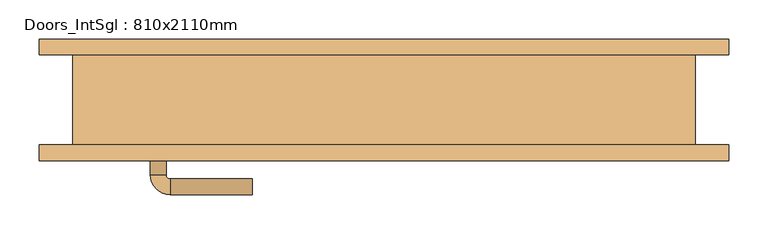
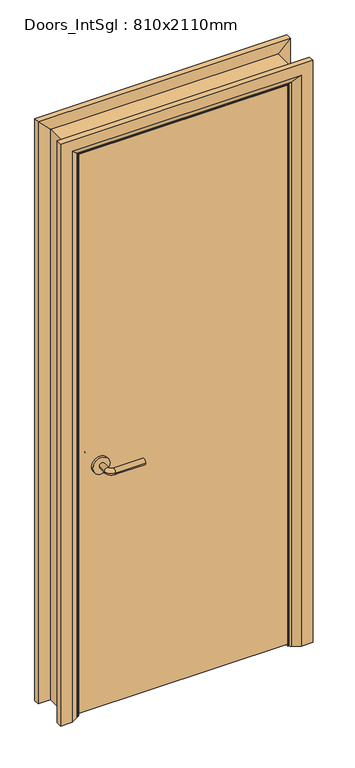
"""IFC4 building model written with IfcOpenShell, lengths in millimetres: door geometry, Doors_IntSgl : 810x2110mm."""

from ifc_helpers import new_model, si_unit, point, frame, frame_2d, origin, place, context, project, spatial, polyline, circle_curve, ellipse_curve, trimmed, segment, composite_curve, outline, extrude, faceted_brep, source, transform, mapped, element, save
from ifc_brep_helpers import plane_surface, cylinder_surface, revolved_surface, advanced_brep


def doors_intsgl_810x2110mm_b7c9fbf7(model_context):
    return source(origin(), model_context, "Body", "SolidModel", [
        advanced_brep(
        [(-298.0, -11.5, 900.0), (-278.0, -11.5, 900.0), (-298.0, 18.5, 900.0), (-278.0, 18.5, 900.0), (-273.0, 23.5, 900.0), (-273.0, 43.5, 900.0), (-168.0, 43.5, 900.0), (-168.0, 23.5, 900.0)],
        [
            (0, 1, circle_curve(frame((-288.0, -11.5, 900.0), z_axis=(0.0, -1.0, 0.0), x_axis=(1.0, 0.0, 0.0)), 10.0)),
            (1, 0, circle_curve(frame((-288.0, -11.5, 900.0), z_axis=(0.0, -1.0, 0.0), x_axis=(1.0, 0.0, 0.0)), 10.0)),
            (0, 2),
            (2, 3, circle_curve(frame((-288.0, 18.5, 900.0), z_axis=(0.0, -1.0, 0.0), x_axis=(1.0, 0.0, 0.0)), 10.0)),
            (3, 1),
            (3, 2, circle_curve(frame((-288.0, 18.5, 900.0), z_axis=(0.0, -1.0, 0.0), x_axis=(1.0, 0.0, 0.0)), 10.0)),
            (4, 3, circle_curve(frame((-273.0, 18.5, 900.0), z_axis=(0.0, 0.0, 1.0), x_axis=(-1.0, 0.0, 0.0)), 5.0)),
            (2, 5, circle_curve(frame((-273.0, 18.5, 900.0), z_axis=(0.0, 0.0, -1.0), x_axis=(-1.0, 0.0, 0.0)), 25.0)),
            (5, 4, circle_curve(frame((-273.0, 33.5, 900.0), z_axis=(-1.0, 0.0, 0.0), x_axis=(0.0, -1.0, 0.0)), 10.0)),
            (4, 5, circle_curve(frame((-273.0, 33.5, 900.0), z_axis=(-1.0, 0.0, 0.0), x_axis=(0.0, -1.0, 0.0)), 10.0)),
            (6, 7, circle_curve(frame((-168.0, 33.5, 900.0), z_axis=(1.0, 0.0, 0.0), x_axis=(0.0, -1.0, 0.0)), 10.0)),
            (7, 6, circle_curve(frame((-168.0, 33.5, 900.0), z_axis=(1.0, 0.0, 0.0), x_axis=(0.0, -1.0, 0.0)), 10.0)),
            (5, 6),
            (7, 4),
        ],
        [
            plane_surface(frame((-288.0, -11.5, 900.0), z_axis=(0.0, -1.0, 0.0), x_axis=(0.0, 0.0, 1.0))),
            cylinder_surface(frame((-288.0, -11.5, 900.0), z_axis=(0.0, -1.0, 0.0), x_axis=(1.0, 0.0, 0.0)), 10.0),
            revolved_surface(trimmed(ellipse_curve(frame((-288.0, 18.5, 900.0), z_axis=(0.0, -1.0, 0.0), x_axis=(1.0, 0.0, 0.0)), 10.0, 10.0), [point((-298.0, 18.5, 900.0))], [point((-278.0, 18.5, 900.0))], True, "CARTESIAN"), (-273.0, 18.5, 900.0), (0.0, 0.0, -1.0)),
            revolved_surface(trimmed(ellipse_curve(frame((-288.0, 18.5, 900.0), z_axis=(0.0, -1.0, 0.0), x_axis=(1.0, 0.0, 0.0)), 10.0, 10.0), [point((-278.0, 18.5, 900.0))], [point((-298.0, 18.5, 900.0))], True, "CARTESIAN"), (-273.0, 18.5, 900.0), (0.0, 0.0, -1.0)),
            plane_surface(frame((-168.0, 33.5, 900.0), z_axis=(1.0, 0.0, 0.0), x_axis=(0.0, 0.0, 1.0))),
            cylinder_surface(frame((-273.0, 33.5, 900.0), z_axis=(-1.0, 0.0, 0.0), x_axis=(0.0, -1.0, 0.0)), 10.0),
        ],
        [
            (0, [[1, 2]]),
            (1, [[-1, 3, 4, 5]]),
            (1, [[-2, -5, 6, -3]]),
            (2, [[7, -4, 8, 9]]),
            (3, [[-8, -6, -7, 10]]),
            (4, [[11, 12]]),
            (5, [[-9, 13, -12, 14]]),
            (5, [[-10, -14, -11, -13]]),
        ],
    ),
        extrude(outline(composite_curve([segment(trimmed(circle_curve(frame_2d((900.0, -290.5)), 30.0), [point((900.0, -320.5))], [point((900.0, -260.5))], False, "CARTESIAN"), True, "CONTINUOUS"), segment(trimmed(circle_curve(frame_2d((900.0, -290.5)), 30.0), [point((900.0, -260.5))], [point((900.0, -320.5))], False, "CARTESIAN"), True, "CONTINUOUS")], self_intersect=False)), frame((0.0, -19.5, 0.0), z_axis=(0.0, 1.0, 0.0), x_axis=(0.0, 0.0, 1.0)), (0.0, 0.0, 1.0), 8.0),
        advanced_brep(
        [(-298.0, -65.5, 900.0), (-278.0, -65.5, 900.0), (-278.0, -95.5, 900.0), (-298.0, -95.5, 900.0), (-273.0, -100.5, 900.0), (-273.0, -120.5, 900.0), (-168.0, -120.5, 900.0), (-168.0, -100.5, 900.0)],
        [
            (0, 1, circle_curve(frame((-288.0, -65.5, 900.0), z_axis=(0.0, 1.0, 0.0), x_axis=(1.0, 0.0, 0.0)), 10.0)),
            (1, 0, circle_curve(frame((-288.0, -65.5, 900.0), z_axis=(0.0, 1.0, 0.0), x_axis=(1.0, 0.0, 0.0)), 10.0)),
            (1, 2),
            (2, 3, circle_curve(frame((-288.0, -95.5, 900.0), z_axis=(0.0, 1.0, 0.0), x_axis=(1.0, 0.0, 0.0)), 10.0)),
            (3, 0),
            (3, 2, circle_curve(frame((-288.0, -95.5, 900.0), z_axis=(0.0, 1.0, 0.0), x_axis=(1.0, 0.0, 0.0)), 10.0)),
            (4, 5, circle_curve(frame((-273.0, -110.5, 900.0), z_axis=(-1.0, 0.0, 0.0), x_axis=(0.0, 1.0, 0.0)), 10.0)),
            (5, 3, circle_curve(frame((-273.0, -95.5, 900.0), z_axis=(0.0, 0.0, -1.0), x_axis=(-1.0, 0.0, 0.0)), 25.0)),
            (2, 4, circle_curve(frame((-273.0, -95.5, 900.0), z_axis=(0.0, 0.0, 1.0), x_axis=(-1.0, 0.0, 0.0)), 5.0)),
            (5, 4, circle_curve(frame((-273.0, -110.5, 900.0), z_axis=(-1.0, 0.0, 0.0), x_axis=(0.0, 1.0, 0.0)), 10.0)),
            (6, 7, circle_curve(frame((-168.0, -110.5, 900.0), z_axis=(1.0, 0.0, 0.0), x_axis=(0.0, 1.0, 0.0)), 10.0)),
            (7, 6, circle_curve(frame((-168.0, -110.5, 900.0), z_axis=(1.0, 0.0, 0.0), x_axis=(0.0, 1.0, 0.0)), 10.0)),
            (4, 7),
            (6, 5),
        ],
        [
            plane_surface(frame((-288.0, -65.5, 900.0), z_axis=(0.0, 1.0, 0.0), x_axis=(0.0, 0.0, 1.0))),
            cylinder_surface(frame((-288.0, -65.5, 900.0), z_axis=(0.0, 1.0, 0.0), x_axis=(1.0, 0.0, 0.0)), 10.0),
            revolved_surface(trimmed(ellipse_curve(frame((-288.0, -95.5, 900.0), z_axis=(0.0, -1.0, 0.0), x_axis=(1.0, 0.0, 0.0)), 10.0, 10.0), [point((-298.0, -95.5, 900.0))], [point((-278.0, -95.5, 900.0))], True, "CARTESIAN"), (-273.0, -95.5, 900.0), (0.0, 0.0, -1.0)),
            revolved_surface(trimmed(ellipse_curve(frame((-288.0, -95.5, 900.0), z_axis=(0.0, -1.0, 0.0), x_axis=(1.0, 0.0, 0.0)), 10.0, 10.0), [point((-278.0, -95.5, 900.0))], [point((-298.0, -95.5, 900.0))], True, "CARTESIAN"), (-273.0, -95.5, 900.0), (0.0, 0.0, -1.0)),
            plane_surface(frame((-168.0, -110.5, 900.0), z_axis=(1.0, 0.0, 0.0), x_axis=(0.0, 0.0, 1.0))),
            cylinder_surface(frame((-273.0, -110.5, 900.0), z_axis=(-1.0, 0.0, 0.0), x_axis=(0.0, 1.0, 0.0)), 10.0),
        ],
        [
            (0, [[1, 2]]),
            (1, [[3, 4, 5, -2]]),
            (1, [[-5, 6, -3, -1]]),
            (2, [[7, 8, -4, 9]]),
            (3, [[10, -9, -6, -8]]),
            (4, [[11, 12]]),
            (5, [[13, -11, 14, -7]]),
            (5, [[-14, -12, -13, -10]]),
        ],
    ),
        extrude(outline(composite_curve([segment(trimmed(circle_curve(frame_2d((900.0, -290.5)), 30.0), [point((900.0, -320.5))], [point((900.0, -260.5))], False, "CARTESIAN"), True, "CONTINUOUS"), segment(trimmed(circle_curve(frame_2d((900.0, -290.5)), 30.0), [point((900.0, -260.5))], [point((900.0, -320.5))], False, "CARTESIAN"), True, "CONTINUOUS")], self_intersect=False)), frame((0.0, -65.5, 0.0), z_axis=(0.0, 1.0, 0.0), x_axis=(0.0, 0.0, 1.0)), (0.0, 0.0, 1.0), 8.0),
        extrude(outline(polyline([(363.0, -19.5), (363.0, -57.5), (-363.0, -57.5), (-363.0, -19.5), (363.0, -19.5)])), frame((0.0, 0.0, 8.0), z_axis=(0.0, 0.0, 1.0), x_axis=(1.0, 0.0, 0.0)), (0.0, 0.0, 1.0), 2060.0),
        advanced_brep(
        [(440.0, -77.5, 0.0), (400.0, -77.5, 0.0), (374.0, -63.5, 0.0), (370.0, -57.5, 0.0), (440.0, -57.5, 0.0), (440.0, -57.5, 2145.0), (440.0, -77.5, 2145.0), (370.0, -57.5, 2075.0), (-370.0, -57.5, 2075.0), (-370.0, -57.5, 0.0), (-440.0, -57.5, 0.0), (-440.0, -57.5, 2145.0), (374.0, -63.5, 2079.0), (400.0, -77.5, 2105.0), (-440.0, -77.5, 2145.0), (-440.0, -77.5, 0.0), (-400.0, -77.5, 0.0), (-400.0, -77.5, 2105.0), (-374.0, -63.5, 2079.0), (-374.0, -63.5, 0.0)],
        [
            (0, 1),
            (1, 2),
            (2, 3, circle_curve(frame((378.0, -56.5, 0.0), z_axis=(0.0, 0.0, -1.0), x_axis=(1.0, 0.0, 0.0)), 8.0622577)),
            (3, 4),
            (4, 0),
            (4, 5),
            (5, 6),
            (6, 0),
            (3, 7),
            (7, 8),
            (8, 9),
            (9, 10),
            (10, 11),
            (11, 5),
            (2, 12),
            (12, 7, ellipse_curve(frame((378.0, -56.5, 2083.0), z_axis=(0.7071067811865475, 0.0, -0.7071067811865475), x_axis=(-0.7071067811865474, 0.0, -0.7071067811865476)), 11.4017543, 8.0622577)),
            (1, 13),
            (13, 12),
            (6, 14),
            (14, 15),
            (15, 16),
            (16, 17),
            (17, 13),
            (11, 14),
            (12, 18),
            (18, 8, ellipse_curve(frame((-378.0, -56.5, 2083.0), z_axis=(0.7071067811865475, 0.0, 0.7071067811865475), x_axis=(0.7071067811865476, 0.0, -0.7071067811865474)), 11.4017543, 8.0622577)),
            (17, 18),
            (15, 10),
            (9, 19, circle_curve(frame((-378.0, -56.5, 0.0), z_axis=(0.0, 0.0, -1.0), x_axis=(-1.0, 0.0, 0.0)), 8.0622577)),
            (19, 16),
            (18, 19),
        ],
        [
            plane_surface(frame((370.0, -57.5, 0.0), z_axis=(0.0, 0.0, -1.0), x_axis=(0.0, 1.0, 0.0))),
            plane_surface(frame((440.0, -77.5, 0.0), z_axis=(1.0, 0.0, 0.0), x_axis=(0.0, 0.0, 1.0))),
            plane_surface(frame((440.0, -57.5, 0.0), z_axis=(0.0, 1.0, 0.0), x_axis=(0.0, 0.0, 1.0))),
            cylinder_surface(frame((378.0, -56.5, 0.0), z_axis=(0.0, 0.0, -1.0), x_axis=(1.0, 0.0, 0.0)), 8.0622577),
            plane_surface(frame((374.0, -63.5, 0.0), z_axis=(-0.4740998230350126, -0.880471099922178, 0.0), x_axis=(0.0, 0.0, 1.0))),
            plane_surface(frame((400.0, -77.5, 0.0), z_axis=(0.0, -1.0, 0.0), x_axis=(0.0, 0.0, 1.0))),
            plane_surface(frame((440.0, -77.5, 2145.0), z_axis=(0.0, 0.0, 1.0), x_axis=(-1.0, 0.0, 0.0))),
            cylinder_surface(frame((370.0, -56.5, 2083.0), z_axis=(1.0, 0.0, 0.0), x_axis=(0.0, 0.0, 1.0)), 8.0622577),
            plane_surface(frame((374.0, -63.5, 2079.0), z_axis=(0.0, -0.8804710999221764, -0.4740998230350154), x_axis=(-1.0, 0.0, 0.0))),
            plane_surface(frame((-370.0, -57.5, 0.0), z_axis=(0.0, 0.0, -1.0), x_axis=(0.0, 1.0, 0.0))),
            plane_surface(frame((-440.0, -77.5, 2145.0), z_axis=(-1.0, 0.0, 0.0), x_axis=(0.0, 0.0, -1.0))),
            cylinder_surface(frame((-378.0, -56.5, 2075.0), z_axis=(0.0, 0.0, 1.0), x_axis=(-1.0, 0.0, 0.0)), 8.0622577),
            plane_surface(frame((-374.0, -63.5, 2079.0), z_axis=(0.47409982303501824, -0.8804710999221749, 0.0), x_axis=(0.0, 0.0, -1.0))),
        ],
        [
            (0, [[1, 2, 3, 4, 5]]),
            (1, [[6, 7, 8, -5]]),
            (2, [[9, 10, 11, 12, 13, 14, -6, -4]]),
            (3, [[15, 16, -9, -3]]),
            (4, [[17, 18, -15, -2]]),
            (5, [[-8, 19, 20, 21, 22, 23, -17, -1]]),
            (6, [[-14, 24, -19, -7]]),
            (7, [[25, 26, -10, -16]]),
            (8, [[-23, 27, -25, -18]]),
            (9, [[28, -12, 29, 30, -21]]),
            (10, [[-13, -28, -20, -24]]),
            (11, [[31, -29, -11, -26]]),
            (12, [[-22, -30, -31, -27]]),
        ],
    ),
        extrude(outline(polyline([(0.0, -346.0), (2051.0, -346.0), (2051.0, 346.0), (0.0, 346.0), (0.0, 365.0), (2070.0, 365.0), (2070.0, -365.0), (0.0, -365.0), (0.0, -346.0)])), frame((0.0, -17.5, 0.0), z_axis=(0.0, 1.0, 0.0), x_axis=(0.0, 0.0, 1.0)), (0.0, 0.0, 1.0), 32.0),
        advanced_brep(
        [(-440.0, 77.5, 0.0), (-400.0, 77.5, 0.0), (-374.0, 63.5, 0.0), (-370.0, 57.5, 0.0), (-440.0, 57.5, 0.0), (-440.0, 57.5, 2145.0), (-440.0, 77.5, 2145.0), (-370.0, 57.5, 2075.0), (-374.0, 63.5, 2079.0), (-400.0, 77.5, 2105.0), (440.0, 57.5, 2145.0), (440.0, 77.5, 2145.0), (370.0, 57.5, 2075.0), (374.0, 63.5, 2079.0), (400.0, 77.5, 2105.0), (440.0, 77.5, 0.0), (440.0, 57.5, 0.0), (370.0, 57.5, 0.0), (374.0, 63.5, 0.0), (400.0, 77.5, 0.0)],
        [
            (0, 1),
            (1, 2),
            (2, 3, circle_curve(frame((-378.0, 56.5, 0.0), z_axis=(0.0, 0.0, -1.0), x_axis=(-1.0, 0.0, 0.0)), 8.0622577)),
            (3, 4),
            (4, 0),
            (4, 5),
            (5, 6),
            (6, 0),
            (3, 7),
            (7, 5),
            (2, 8),
            (8, 7, ellipse_curve(frame((-378.0, 56.5, 2083.0), z_axis=(-0.7071067811865475, 0.0, -0.7071067811865475), x_axis=(0.7071067811865474, 0.0, -0.7071067811865476)), 11.4017543, 8.0622577)),
            (1, 9),
            (9, 8),
            (6, 9),
            (5, 10),
            (10, 11),
            (11, 6),
            (7, 12),
            (12, 10),
            (8, 13),
            (13, 12, ellipse_curve(frame((378.0, 56.5, 2083.0), z_axis=(-0.7071067811865475, 0.0, 0.7071067811865475), x_axis=(-0.7071067811865476, 0.0, -0.7071067811865474)), 11.4017543, 8.0622577)),
            (9, 14),
            (14, 13),
            (11, 14),
            (15, 16),
            (16, 17),
            (17, 18, circle_curve(frame((378.0, 56.5, 0.0), z_axis=(0.0, 0.0, -1.0), x_axis=(1.0, 0.0, 0.0)), 8.0622577)),
            (18, 19),
            (19, 15),
            (10, 16),
            (15, 11),
            (12, 17),
            (13, 18),
            (14, 19),
        ],
        [
            plane_surface(frame((-370.0, 130.3010989, 0.0), z_axis=(0.0, 0.0, -1.0), x_axis=(1.0, 0.0, 0.0))),
            plane_surface(frame((-440.0, 77.5, 0.0), z_axis=(-1.0, 0.0, 0.0), x_axis=(0.0, 0.0, 1.0))),
            plane_surface(frame((-440.0, 57.5, 0.0), z_axis=(0.0, -1.0, 0.0), x_axis=(0.0, 0.0, 1.0))),
            cylinder_surface(frame((-378.0, 56.5, 0.0), z_axis=(0.0, 0.0, -1.0), x_axis=(-1.0, 0.0, 0.0)), 8.0622577),
            plane_surface(frame((-374.0, 63.5, 0.0), z_axis=(0.4740998230350183, 0.8804710999221749, 0.0), x_axis=(0.0, 0.0, 1.0))),
            plane_surface(frame((-400.0, 77.5, 0.0), z_axis=(0.0, 1.0, 0.0), x_axis=(0.0, 0.0, 1.0))),
            plane_surface(frame((-440.0, 77.5, 2145.0), z_axis=(0.0, 0.0, 1.0), x_axis=(1.0, 0.0, 0.0))),
            plane_surface(frame((-440.0, 57.5, 2145.0), z_axis=(0.0, -1.0, 0.0), x_axis=(1.0, 0.0, 0.0))),
            cylinder_surface(frame((-370.0, 56.5, 2083.0), z_axis=(-1.0, 0.0, 0.0), x_axis=(0.0, 0.0, 1.0)), 8.0622577),
            plane_surface(frame((-374.0, 63.5, 2079.0), z_axis=(0.0, 0.8804710999221749, -0.4740998230350183), x_axis=(1.0, 0.0, 0.0))),
            plane_surface(frame((-400.0, 77.5, 2105.0), z_axis=(0.0, 1.0, 0.0), x_axis=(1.0, 0.0, 0.0))),
            plane_surface(frame((370.0, 130.3010989, 0.0), z_axis=(0.0, 0.0, -1.0), x_axis=(-1.0, 0.0, 0.0))),
            plane_surface(frame((440.0, 77.5, 2145.0), z_axis=(1.0, 0.0, 0.0), x_axis=(0.0, 0.0, -1.0))),
            plane_surface(frame((440.0, 57.5, 2145.0), z_axis=(0.0, -1.0, 0.0), x_axis=(0.0, 0.0, -1.0))),
            cylinder_surface(frame((378.0, 56.5, 2075.0), z_axis=(0.0, 0.0, 1.0), x_axis=(1.0, 0.0, 0.0)), 8.0622577),
            plane_surface(frame((374.0, 63.5, 2079.0), z_axis=(-0.4740998230350183, 0.8804710999221749, 0.0), x_axis=(0.0, 0.0, -1.0))),
            plane_surface(frame((400.0, 77.5, 2105.0), z_axis=(0.0, 1.0, 0.0), x_axis=(0.0, 0.0, -1.0))),
        ],
        [
            (0, [[1, 2, 3, 4, 5]]),
            (1, [[6, 7, 8, -5]]),
            (2, [[9, 10, -6, -4]]),
            (3, [[11, 12, -9, -3]]),
            (4, [[13, 14, -11, -2]]),
            (5, [[-8, 15, -13, -1]]),
            (6, [[16, 17, 18, -7]]),
            (7, [[19, 20, -16, -10]]),
            (8, [[21, 22, -19, -12]]),
            (9, [[23, 24, -21, -14]]),
            (10, [[-18, 25, -23, -15]]),
            (11, [[26, 27, 28, 29, 30]]),
            (12, [[31, -26, 32, -17]]),
            (13, [[33, -27, -31, -20]]),
            (14, [[34, -28, -33, -22]]),
            (15, [[35, -29, -34, -24]]),
            (16, [[-32, -30, -35, -25]]),
        ],
    ),
        faceted_brep([(-365.0, -57.5, 0.0), (-397.0, -57.5, 0.0), (-397.0, 57.5, 0.0), (-365.0, 57.5, 0.0), (-365.0, 57.5, 2070.0), (-365.0, -57.5, 2070.0), (-397.0, 57.5, 2102.0), (-397.0, -57.5, 2102.0), (365.0, 57.5, 2070.0), (365.0, -57.5, 2070.0), (397.0, 57.5, 2102.0), (397.0, -57.5, 2102.0), (365.0, -57.5, 0.0), (365.0, 57.5, 0.0), (397.0, 57.5, 0.0), (397.0, -57.5, 0.0)], [[[0, 1, 2, 3]], [[3, 4, 5, 0]], [[2, 6, 4, 3]], [[1, 7, 6, 2]], [[0, 5, 7, 1]], [[4, 8, 9, 5]], [[6, 10, 8, 4]], [[7, 11, 10, 6]], [[5, 9, 11, 7]], [[12, 13, 14, 15]], [[8, 13, 12, 9]], [[10, 14, 13, 8]], [[11, 15, 14, 10]], [[9, 12, 15, 11]]]),
    ])


if __name__ == "__main__":
    model = new_model("IFC4")
    model_context = context("Model", 3, world=origin())
    ifc_project = project(units=[si_unit("LENGTHUNIT", "METRE", prefix="MILLI")], contexts=[model_context])
    site = spatial("IfcSite", under=ifc_project)
    building = spatial("IfcBuilding", under=site)
    placement = place(None, origin())
    doors_intsgl_810x2110mm_shape = doors_intsgl_810x2110mm_b7c9fbf7(model_context)
    element("IfcDoor", 1, ObjectType="Doors_IntSgl : 810x2110mm", at=placement, inside=building, context=model_context, shape_type="MappedRepresentation", body=[
        mapped(doors_intsgl_810x2110mm_shape, transform((0.0, 0.0, 0.0), x_axis=(1.0, 0.0, 0.0), y_axis=(0.0, 1.0, 0.0), z_axis=(0.0, 0.0, 1.0))),
    ])
    save(model, "model.ifc")

# Revit data of these elements
# Type "Doors_IntSgl : 810x2110mm"
#   Construction Type Id = "MDOOR"
#   Type Mark = "42"
#   Type Comments = "Internal Single"
#   Operation = "SingleSwingRight"
#   Manufacturer = "Revit"
#   Keynote = "L20"
#   Description = "Internal Single Door"
#   Analytic Construction = "Metal"
#   UnderCut = 8 mm
#   Tolerance = 2 mm
#   Thickness = 38 mm
#   Thermal Resistance (R) = 0.270117 (m²·K)/W
#   Structural Tolerance = 8 mm
#   StopDepth = 32 mm
#   Stop Thickness = 19 mm
#   Rough Width = 810 mm
#   Rough Height = 2110 mm
#   Height to Top Lock Rail = 1000 mm
#   Heat Transfer Coefficient (U) = 3.7021 W/(m²·K)
#   Handle Z Distance = 900 mm
#   Handle X Distance = 75 mm
#   Frame Thickness = 32 mm
#   Door Panel Width = 726 mm
#   Door Panel Thickness = 38 mm
#   Door Panel Offset = 0 mm
#   Height = 2110 mm
#   Width = 810 mm
#   Door Panel Height = 2060 mm
#   Architrave Setback = 5 mm
#   Define Thermal Properties by = 1
#   Vis - Ironmongery = yes
#   Material Ironmongery = Door - Handle
#   Material Frame = Door - Frame/Mullion (1)
#   Material Door = Door - Panel
#   Material Architrave = Door - Architrave
#   Visual Light Transmittance = 0
#   Solar Heat Gain Coefficient = 0
#   Function = (empty or 0)
#   Wall Closure = (empty or 0)
# Element 1 (IfcDoor, "Doors_IntSgl : 810x2110mm")
#   Materials on its faces: "Door - Architrave", "Door - Handle", "Door - Frame/Mullion (1)", "Door - Panel"
# Materials
#   "Door - Handle": class "Miscellaneous", colour RGB 0 0 0, transparency 0, Keynote = "P21", Cost = 0
#   "Door - Frame/Mullion (1)": class "Wood", colour RGB 212 179 113, transparency 0, Keynote = "L20", Cost = 0
#   "Door - Panel": class "Wood", colour RGB 210 159 95, transparency 0, Keynote = "L20", Cost = 0
#   "Door - Architrave": class "Wood", colour RGB 154 90 5, transparency 0, Keynote = "P20", Cost = 0
